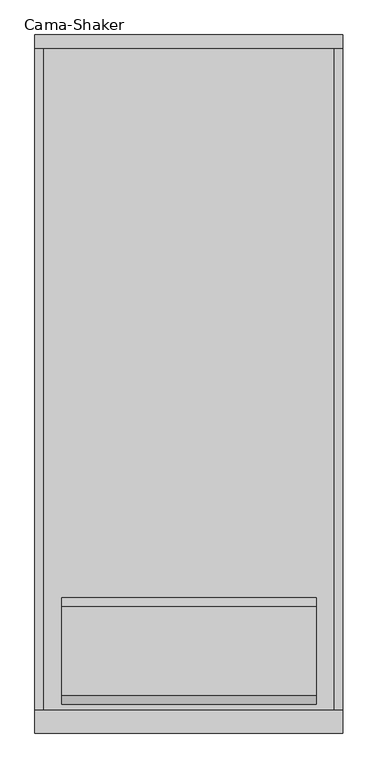
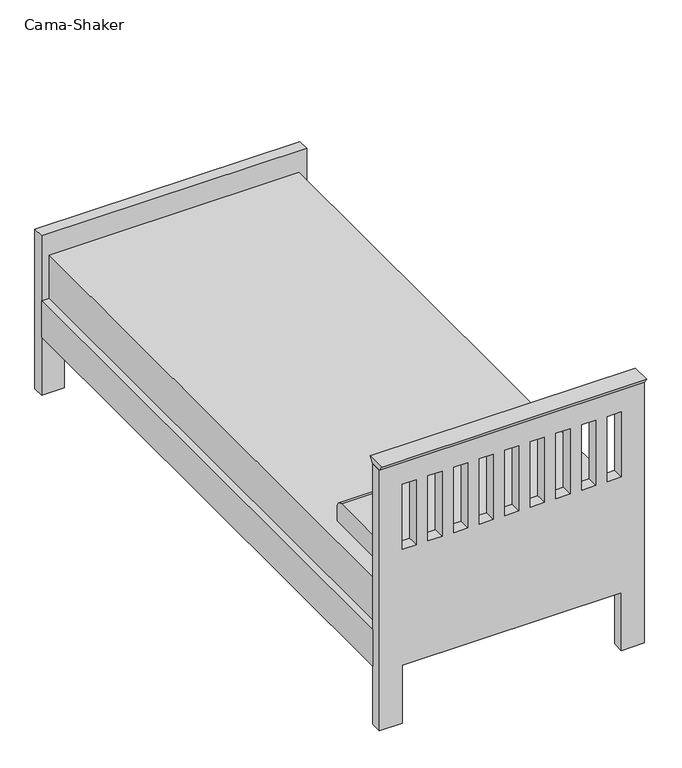
"""IFC4 building model written with IfcOpenShell, lengths in millimetres: furniture geometry, Cama-Shaker : 880 x 1981 mm - Solteiro."""

from ifc_helpers import new_model, si_unit, point, frame, frame_2d, origin, place, context, project, spatial, polyline, circle_curve, trimmed, segment, composite_curve, outline, extrude, source, transform, mapped, element, save


def cama_shaker_46b0d072(model_context):
    return source(origin(), model_context, "Body", "SweptSolid", [
        extrude(outline(polyline([(38.1, 914.4), (0.0, 914.4), (-13.8545455, 933.45), (51.9545455, 933.45), (38.1, 914.4)])), frame((-458.8365546, 0.0, 0.0), z_axis=(1.0, 0.0, 0.0), x_axis=(0.0, 1.0, 0.0)), (0.0, 0.0, 1.0), 880.0533613),
        extrude(outline(composite_curve([segment(polyline([(373.2486637, 482.6), (68.4486637, 482.6), (68.4486637, 533.4)]), True, "CONTINUOUS"), segment(trimmed(circle_curve(frame_2d((93.8486637, 533.4)), 25.4), [point((68.4486637, 533.4))], [point((93.8486637, 558.8))], False, "CARTESIAN"), True, "CONTINUOUS"), segment(polyline([(93.8486637, 558.8), (347.8486637, 558.8)]), True, "CONTINUOUS"), segment(trimmed(circle_curve(frame_2d((347.8486637, 533.4)), 25.4), [point((347.8486637, 558.8))], [point((373.2486637, 533.4))], False, "CARTESIAN"), True, "CONTINUOUS"), segment(polyline([(373.2486637, 533.4), (373.2486637, 482.6)]), True, "CONTINUOUS")], self_intersect=False)), frame((-382.85, 0.0, 0.0), z_axis=(1.0, 0.0, 0.0), x_axis=(0.0, 1.0, 0.0)), (0.0, 0.0, 1.0), 727.6),
        extrude(outline(polyline([(395.55, 38.1), (-433.65, 38.1), (-433.65, 1943.1), (395.55, 1943.1), (395.55, 38.1)])), frame((0.0, 0.0, 228.6), z_axis=(0.0, 0.0, 1.0), x_axis=(1.0, 0.0, 0.0)), (0.0, 0.0, 1.0), 254.0),
        extrude(outline(polyline([(395.55, 1943.1), (420.95, 1943.1), (420.95, 38.1), (395.55, 38.1), (395.55, 1943.1)])), frame((0.0, 0.0, 203.0994861), z_axis=(0.0, 0.0, 1.0), x_axis=(1.0, 0.0, 0.0)), (0.0, 0.0, 1.0), 127.0),
        extrude(outline(polyline([(-459.05, 1943.1), (-433.65, 1943.1), (-433.65, 38.1), (-459.05, 38.1), (-459.05, 1943.1)])), frame((0.0, 0.0, 203.5755296), z_axis=(0.0, 0.0, 1.0), x_axis=(1.0, 0.0, 0.0)), (0.0, 0.0, 1.0), 127.0),
        extrude(outline(polyline([(0.0, -382.85), (203.2, -382.85), (203.2, 344.75), (0.0, 344.75), (0.0, 420.95), (558.8, 420.95), (558.8, -459.05), (0.0, -459.05), (0.0, -382.85)])), frame((0.0, 1943.1, 0.0), z_axis=(0.0, 1.0, 0.0), x_axis=(0.0, 0.0, 1.0)), (0.0, 0.0, 1.0), 38.1),
        extrude(outline(polyline([(914.4, 421.2168067), (914.4, -458.8365546), (0.0, -458.8365546), (0.0, -382.85), (203.2, -382.85), (203.2, 344.75), (0.0, 344.75), (0.0, 421.2168067), (914.4, 421.2168067)]), holes=[polyline([(838.2, -335.8722222), (609.6, -335.8722222), (609.6, -382.85), (838.2, -382.85), (838.2, -335.8722222)]), polyline([(838.2, -250.7944444), (609.6, -250.7944444), (609.6, -297.7722222), (838.2, -297.7722222), (838.2, -250.7944444)]), polyline([(838.2, -165.7166667), (609.6, -165.7166667), (609.6, -212.6944444), (838.2, -212.6944444), (838.2, -165.7166667)]), polyline([(838.2, -80.6388889), (609.6, -80.6388889), (609.6, -127.6166667), (838.2, -127.6166667), (838.2, -80.6388889)]), polyline([(838.2, 89.5166667), (609.6, 89.5166667), (609.6, 42.5388889), (838.2, 42.5388889), (838.2, 89.5166667)]), polyline([(838.2, 174.5944444), (609.6, 174.5944444), (609.6, 127.6166667), (838.2, 127.6166667), (838.2, 174.5944444)]), polyline([(838.2, 259.6722222), (609.6, 259.6722222), (609.6, 212.6944444), (838.2, 212.6944444), (838.2, 259.6722222)]), polyline([(838.2, 344.75), (609.6, 344.75), (609.6, 297.7722222), (838.2, 297.7722222), (838.2, 344.75)]), polyline([(838.2, 4.4388889), (609.6, 4.4388889), (609.6, -42.5388889), (838.2, -42.5388889), (838.2, 4.4388889)])]), frame((0.0, 0.0, 0.0), z_axis=(0.0, 1.0, 0.0), x_axis=(0.0, 0.0, 1.0)), (0.0, 0.0, 1.0), 38.1),
    ])


if __name__ == "__main__":
    model = new_model("IFC4")
    model_context = context("Model", 3, world=origin())
    ifc_project = project(units=[si_unit("LENGTHUNIT", "METRE", prefix="MILLI")], contexts=[model_context])
    site = spatial("IfcSite", under=ifc_project)
    building = spatial("IfcBuilding", under=site)
    placement = place(None, origin())
    cama_shaker_shape = cama_shaker_46b0d072(model_context)
    element("IfcFurniture", 1, ObjectType="Cama-Shaker : 880 x 1981 mm - Solteiro", at=placement, inside=building, context=model_context, shape_type="MappedRepresentation", body=[
        mapped(cama_shaker_shape, transform((0.0, 0.0, 0.0), x_axis=(1.0, 0.0, 0.0), y_axis=(0.0, 1.0, 0.0), z_axis=(0.0, 0.0, 1.0))),
    ])
    save(model, "model.ifc")

# Revit data of these elements
# Type "Cama-Shaker : 880 x 1981 mm - Solteiro"
#   Comprimento = 1.9812 m
#   Largura = 0.88 m
#   Material da moldura = wood brown
#   Material do colchão = Linho, branco
# Element 1 (IfcFurniture, "Cama-Shaker : 880 x 1981 mm - Solteiro")
#   Materials on its faces: "wood brown", "Linho, branco"
# Materials
#   "wood brown": class "Wood", colour RGB 80 39 12, transparency 0, Cost = 0
#   "Linho, branco": class "Tecido", colour RGB 247 247 239, transparency 0, Description = "Linho, branco", Cost = 0
